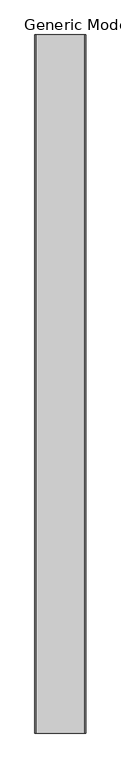
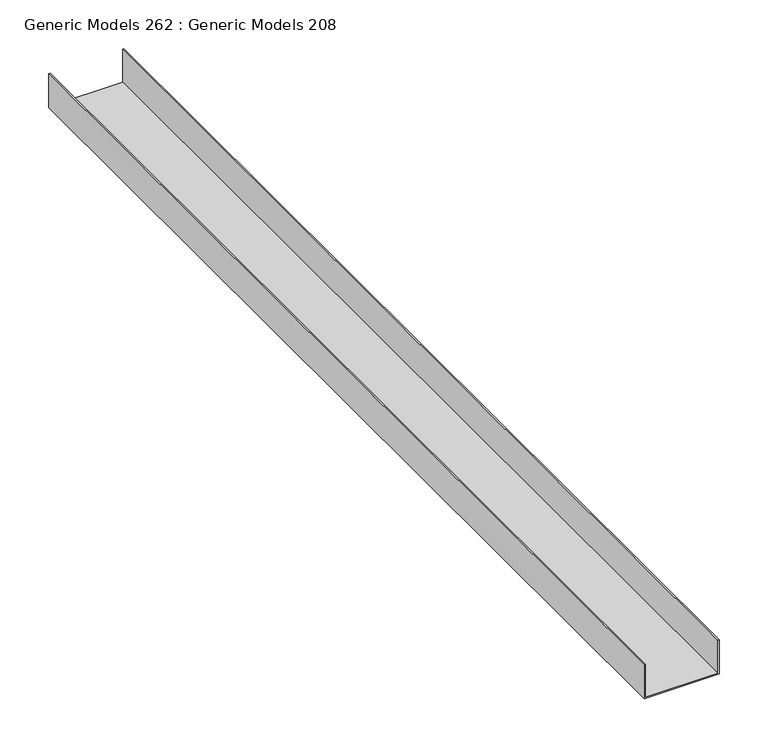
"""IFC4 building model written with IfcOpenShell, lengths in millimetres: proxy geometry, Generic Models 262 : Generic Models 208."""

from ifc_helpers import new_model, si_unit, frame, origin, place, context, project, spatial, polyline, outline, extrude, source, transform, mapped, element, save


def generic_models_262_generic_models_208_e9f11c82(model_context):
    return source(origin(), model_context, "Body", "SweptSolid", [
        extrude(outline(polyline([(2085.2421268, 55683.9204676), (2085.2421268, 55682.3329676), (2042.3796268, 55682.3329676), (2042.3796268, 55771.2329676), (2085.2421268, 55771.2329676), (2085.2421268, 55769.6454676), (2043.9671268, 55769.6454676), (2043.9671268, 55683.9204676), (2085.2421268, 55683.9204676)])), frame((0.0, -228.7033818, 0.0), z_axis=(0.0, 1.0, 0.0), x_axis=(0.0, 0.0, 1.0)), (0.0, 0.0, 1.0), 1219.2),
    ])


if __name__ == "__main__":
    model = new_model("IFC4")
    model_context = context("Model", 3, world=origin())
    ifc_project = project(units=[si_unit("LENGTHUNIT", "METRE", prefix="MILLI")], contexts=[model_context])
    site = spatial("IfcSite", under=ifc_project)
    building = spatial("IfcBuilding", under=site)
    placement = place(None, origin())
    generic_models_262_generic_models_208_shape = generic_models_262_generic_models_208_e9f11c82(model_context)
    element("IfcBuildingElementProxy", 1, Name="Generic Models 262 : Generic Models 208", ObjectType="Generic Models 262 : Generic Models 208", at=placement, inside=building, context=model_context, shape_type="MappedRepresentation", body=[
        mapped(generic_models_262_generic_models_208_shape, transform((0.0, 0.0, 0.0), x_axis=(1.0, 0.0, 0.0), y_axis=(0.0, 1.0, 0.0), z_axis=(0.0, 0.0, 1.0))),
    ])
    save(model, "model.ifc")

# Revit data of these elements
# Element 1 (IfcBuildingElementProxy, "Generic Models 262 : Generic Models 208")
#   Materials on its faces: "METAL STUD CAP"
# Materials
#   "METAL STUD CAP": class "Metal", colour RGB 244 244 244, transparency 0, Description = "Aluminum 6061", Cost = 0
